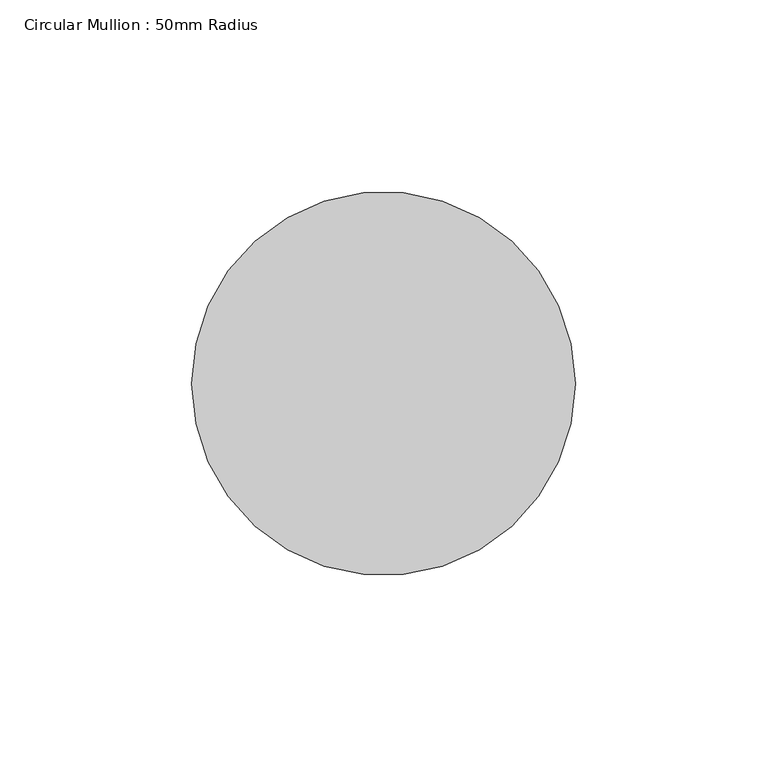
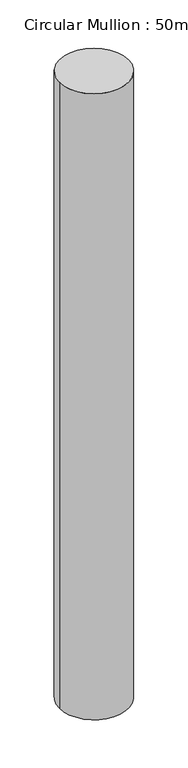
"""IFC4 building model written with IfcOpenShell, lengths in millimetres: member geometry, Circular Mullion : 50mm Radius."""

from ifc_helpers import new_model, si_unit, point, frame, origin, origin_2d, place, context, project, spatial, circle_curve, trimmed, segment, composite_curve, outline, extrude, source, transform, mapped, element, save


def circular_mullion_50mm_radius_84f497e7(model_context):
    return source(origin(), model_context, "Body", "SweptSolid", [
        extrude(outline(composite_curve([segment(trimmed(circle_curve(origin_2d(), 50.0), [point((50.0, 0.0))], [point((-50.0, 0.0))], False, "CARTESIAN"), True, "CONTINUOUS"), segment(trimmed(circle_curve(origin_2d(), 50.0), [point((-50.0, 0.0))], [point((50.0, 0.0))], False, "CARTESIAN"), True, "CONTINUOUS")], self_intersect=False)), frame((0.0, 0.0, -959.8718848), z_axis=(0.0, 0.0, 1.0), x_axis=(1.0, 0.0, 0.0)), (0.0, 0.0, 1.0), 959.8718848),
    ])


if __name__ == "__main__":
    model = new_model("IFC4")
    model_context = context("Model", 3, world=origin())
    ifc_project = project(units=[si_unit("LENGTHUNIT", "METRE", prefix="MILLI")], contexts=[model_context])
    site = spatial("IfcSite", under=ifc_project)
    building = spatial("IfcBuilding", under=site)
    placement = place(None, origin())
    circular_mullion_50mm_radius_shape = circular_mullion_50mm_radius_84f497e7(model_context)
    element("IfcMember", 1, ObjectType="Circular Mullion : 50mm Radius", at=placement, inside=building, context=model_context, shape_type="MappedRepresentation", body=[
        mapped(circular_mullion_50mm_radius_shape, transform((0.0, 0.0, 0.0), x_axis=(1.0, 0.0, 0.0), y_axis=(0.0, 1.0, 0.0), z_axis=(0.0, 0.0, 1.0))),
    ])
    save(model, "model.ifc")

# Revit data of these elements
# Type "Circular Mullion : 50mm Radius"
#   built-in parameter 1007350 = 0.164042 (stored number, unit not read)
# Element 1 (IfcMember, "Circular Mullion : 50mm Radius")
#   Materials on its faces: "Aluminium"
# Materials
#   "Aluminium": class "Metal", colour RGB 247 247 247, transparency 0, Description = "Aluminium 6061", Cost = 0
